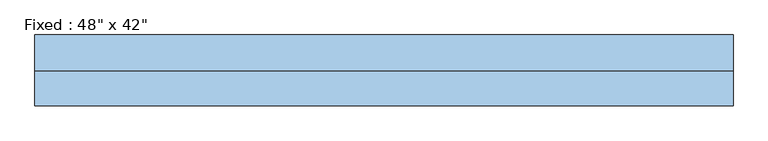
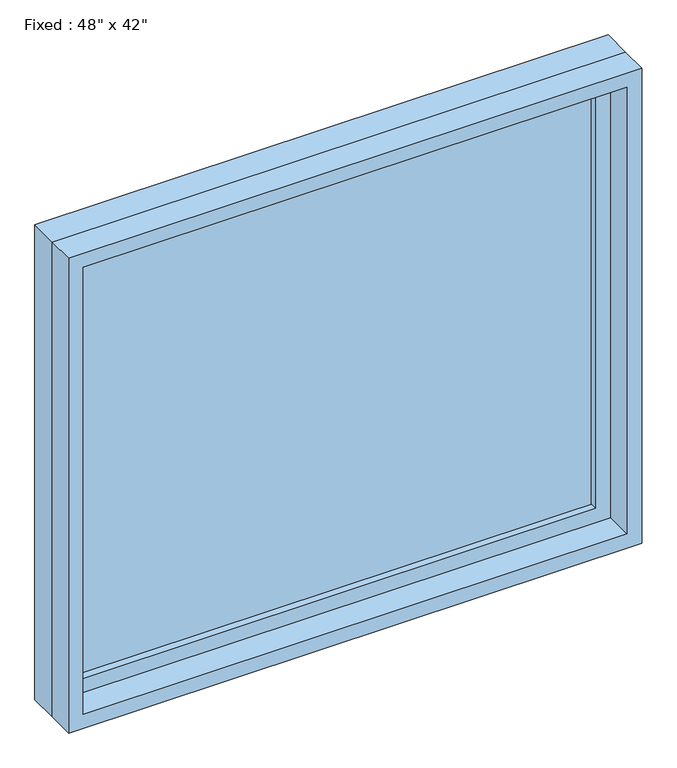
"""IFC4 building model written with IfcOpenShell, lengths in millimetres: window geometry."""

import ifcopenshell
import ifcopenshell.guid

model = None  # the IFC model being written
_history = None  # IfcOwnerHistory: only IFC2X3 demands one
_inside = {}  # id of a spatial element -> (the spatial element, [elements in it])
_under = {}  # id of a project, library or spatial element -> (it, [spatial elements below it])
_declared = {}  # id of a project -> (the project, [libraries it declares])
_typed = {}  # id of a type object -> (the type object, [elements of that type])
_made_of = {}  # id of a material, layer set ... -> (it, [elements and type objects made of it])


def new_model(schema):
    """Start an empty IFC model of exactly this schema.

    Asked for "IFC4X3", IfcOpenShell would pick the latest addendum, in which some entities
    have other attributes; the version numbers below select the first issue.
    IFC2X3 requires an IfcOwnerHistory on every rooted entity: one is made here for all.
    """
    global model, _history
    if schema == "IFC4X3":
        model = ifcopenshell.file(schema_version=(4, 3, 0, 0))
    else:
        model = ifcopenshell.file(schema=schema)
    _inside.clear()
    _under.clear()
    _declared.clear()
    _typed.clear()
    _made_of.clear()
    _history = None
    if model.schema == "IFC2X3":
        org = make("IfcOrganization", Name="unknown")
        user = make(
            "IfcPersonAndOrganization",
            ThePerson=make("IfcPerson", FamilyName="unknown"),
            TheOrganization=org,
        )
        app = make(
            "IfcApplication",
            ApplicationDeveloper=org,
            Version="unknown",
            ApplicationFullName="unknown",
            ApplicationIdentifier="unknown",
        )
        _history = make(
            "IfcOwnerHistory",
            OwningUser=user,
            OwningApplication=app,
            ChangeAction="ADDED",
            CreationDate=0,
        )
    return model


def make(cls, **values):
    """One entity of the class cls with the attributes given. An attribute that is None is left unset."""
    return model.create_entity(
        cls, **{name: value for name, value in values.items() if value is not None}
    )


def rooted(cls, **values):
    """An entity with a GlobalId (a new one), such as an element, a storey or a relation."""
    return make(cls, GlobalId=ifcopenshell.guid.new(), OwnerHistory=_history, **values)


def si_unit(unit_type, name, prefix=None):
    """IfcSIUnit, for example si_unit("LENGTHUNIT", "METRE", prefix="MILLI")."""
    return make("IfcSIUnit", UnitType=unit_type, Prefix=prefix, Name=name)


def assignment(units):
    """IfcUnitAssignment: the units of a project."""
    return None if units is None else make("IfcUnitAssignment", Units=units)


def point(xyz):
    """IfcCartesianPoint."""
    return None if xyz is None else make("IfcCartesianPoint", Coordinates=xyz)


def direction(xyz):
    """IfcDirection."""
    return None if xyz is None else make("IfcDirection", DirectionRatios=xyz)


def frame(location, z_axis=None, x_axis=None):
    """IfcAxis2Placement3D, a coordinate frame: its origin and axes. An axis left out is left unset."""
    return make(
        "IfcAxis2Placement3D",
        Location=point(location),
        Axis=direction(z_axis),
        RefDirection=direction(x_axis),
    )


def origin():
    """The frame at (0, 0, 0) with its axes left unset."""
    return frame((0.0, 0.0, 0.0))


def place(relative_to, where):
    """IfcLocalPlacement: puts the frame where relative to a parent placement (None: the world)."""
    return make(
        "IfcLocalPlacement", PlacementRelTo=relative_to, RelativePlacement=where
    )


def context(
    kind, dimensions, precision=None, world=None, true_north=None, identifier=None
):
    """IfcGeometricRepresentationContext, for example the 3D "Model" context."""
    return make(
        "IfcGeometricRepresentationContext",
        ContextIdentifier=identifier,
        ContextType=kind,
        CoordinateSpaceDimension=dimensions,
        Precision=precision,
        WorldCoordinateSystem=world,
        TrueNorth=true_north,
    )


def project(units=None, contexts=None):
    """IfcProject with its units and contexts."""
    return rooted(
        "IfcProject",
        Name="project",
        RepresentationContexts=contexts,
        UnitsInContext=assignment(units),
    )


def spatial(cls, under=None, at=None, **own):
    """A site, building, storey or space (cls), placed at a placement, below another one or the project."""
    s = rooted(cls, ObjectPlacement=at, **own)
    if under is not None:
        _under.setdefault(under.id(), (under, []))[1].append(s)
    return s


def polyline(points):
    """IfcPolyline through the points."""
    return make("IfcPolyline", Points=[point(p) for p in points])


def outline(outer, holes=None, kind="AREA"):
    """IfcArbitraryClosedProfileDef: a profile drawn as a closed curve; with holes, ...WithVoids."""
    if holes is None:
        return make("IfcArbitraryClosedProfileDef", ProfileType=kind, OuterCurve=outer)
    return make(
        "IfcArbitraryProfileDefWithVoids",
        ProfileType=kind,
        OuterCurve=outer,
        InnerCurves=holes,
    )


def extrude(swept, where, along, depth):
    """IfcExtrudedAreaSolid: the profile swept, set in the frame where, extruded along a direction by depth."""
    return make(
        "IfcExtrudedAreaSolid",
        SweptArea=swept,
        Position=where,
        ExtrudedDirection=direction(along),
        Depth=depth,
    )


def shape(context_of_items, identifier, shape_type, items):
    """IfcShapeRepresentation: the items that make up one representation, for example the "Body"."""
    return make(
        "IfcShapeRepresentation",
        ContextOfItems=context_of_items,
        RepresentationIdentifier=identifier,
        RepresentationType=shape_type,
        Items=items,
    )


def source(mapping_origin, context_of_items, identifier, shape_type, items):
    """IfcRepresentationMap: a shape defined once, which mapped items show again and again."""
    return make(
        "IfcRepresentationMap",
        MappingOrigin=mapping_origin,
        MappedRepresentation=shape(context_of_items, identifier, shape_type, items),
    )


def transform(
    local_origin,
    x_axis=None,
    y_axis=None,
    z_axis=None,
    scale=None,
    scale2=None,
    scale3=None,
    uniform=True,
):
    """IfcCartesianTransformationOperator3D, or its non-uniform kind. x_axis, y_axis, z_axis: its Axis1, 2, 3."""
    if uniform:
        return make(
            "IfcCartesianTransformationOperator3D",
            Axis1=direction(x_axis),
            Axis2=direction(y_axis),
            LocalOrigin=point(local_origin),
            Scale=scale,
            Axis3=direction(z_axis),
        )
    return make(
        "IfcCartesianTransformationOperator3DnonUniform",
        Axis1=direction(x_axis),
        Axis2=direction(y_axis),
        LocalOrigin=point(local_origin),
        Scale=scale,
        Axis3=direction(z_axis),
        Scale2=scale2,
        Scale3=scale3,
    )


def mapped(mapping_source, mapping_target):
    """IfcMappedItem: shows the shape of a source again, moved by a transform."""
    return make(
        "IfcMappedItem", MappingSource=mapping_source, MappingTarget=mapping_target
    )


def made_of(thing, what):
    """Note that an element or type object is made of a material, layer set ...; save() writes the relation."""
    if what is not None:
        _made_of.setdefault(what.id(), (what, []))[1].append(thing)
    return thing


def element(
    cls,
    number,
    at=None,
    inside=None,
    cuts=None,
    type_object=None,
    material=None,
    context=None,
    identifier="Body",
    shape_type=None,
    held_by="IfcProductDefinitionShape",
    body=None,
    shapes=None,
    **own,
):
    """One element of the class cls, such as IfcWall. Its Tag is "e" and its number.

    at: its placement. inside: the storey or other place that contains it. cuts: it is an
    opening in that element (IfcRelVoidsElement). A single representation is given by context,
    identifier, shape_type and body (its items); several are given by shapes. held_by: the class
    of the entity that holds the representations. save() writes the other relations.
    """
    e = rooted(cls, Tag="e%d" % number, ObjectPlacement=at, **own)
    if body is not None:
        shapes = [shape(context, identifier, shape_type, body)]
    if shapes is not None:
        e.Representation = make(held_by, Representations=shapes)
    if inside is not None:
        _inside.setdefault(inside.id(), (inside, []))[1].append(e)
    if cuts is not None:
        rooted(
            "IfcRelVoidsElement", RelatingBuildingElement=cuts, RelatedOpeningElement=e
        )
    if type_object is not None:
        _typed.setdefault(type_object.id(), (type_object, []))[1].append(e)
    return made_of(e, material)


def aggregate(whole, parts):
    """IfcRelAggregates: a whole, such as a stair, and the parts it consists of."""
    return rooted("IfcRelAggregates", RelatingObject=whole, RelatedObjects=parts)


def save(model, path):
    """Write the relations noted so far, then the file.

    IfcRelAggregates (storeys below a building ...), IfcRelContainedInSpatialStructure (elements
    in a storey), IfcRelDefinesByType, IfcRelAssociatesMaterial and IfcRelDeclares: one each for
    every whole, place, type object, material and project.
    """
    for whole, parts in _under.values():
        aggregate(whole, parts)
    for where, things in _inside.values():
        rooted(
            "IfcRelContainedInSpatialStructure",
            RelatedElements=things,
            RelatingStructure=where,
        )
    for kind, things in _typed.values():
        rooted("IfcRelDefinesByType", RelatedObjects=things, RelatingType=kind)
    for what, things in _made_of.values():
        rooted("IfcRelAssociatesMaterial", RelatedObjects=things, RelatingMaterial=what)
    for by, libraries in _declared.values():
        rooted("IfcRelDeclares", RelatingContext=by, RelatedDefinitions=libraries)
    model.write(path)


def window_b58e5159(model_context):
    return source(origin(), model_context, "Body", "SweptSolid", [
        extrude(outline(polyline([(508.0, 14.2875), (-584.2, 14.2875), (-584.2, 26.9875), (508.0, 26.9875), (508.0, 14.2875)])), frame((0.0, 0.0, 977.9), z_axis=(0.0, 0.0, 1.0), x_axis=(1.0, 0.0, 0.0)), (0.0, 0.0, 1.0), 939.8),
        extrude(outline(polyline([(1962.15, -628.65), (933.45, -628.65), (933.45, 552.45), (1962.15, 552.45), (1962.15, -628.65)]), holes=[polyline([(1917.7, -584.2), (1917.7, 508.0), (977.9, 508.0), (977.9, -584.2), (1917.7, -584.2)])]), frame((0.0, -1.5875, 0.0), z_axis=(0.0, 1.0, 0.0), x_axis=(0.0, 0.0, 1.0)), (0.0, 0.0, 1.0), 44.45),
        extrude(outline(polyline([(1981.2, -647.7), (914.4, -647.7), (914.4, 571.5), (1981.2, 571.5), (1981.2, -647.7)]), holes=[polyline([(1949.45, -615.95), (1949.45, 539.75), (946.15, 539.75), (946.15, -615.95), (1949.45, -615.95)])]), frame((0.0, -61.9125, 0.0), z_axis=(0.0, 1.0, 0.0), x_axis=(0.0, 0.0, 1.0)), (0.0, 0.0, 1.0), 60.325),
        extrude(outline(polyline([(1981.2, 571.5), (1981.2, -647.7), (914.4, -647.7), (914.4, 571.5), (1981.2, 571.5)]), holes=[polyline([(1962.15, 552.45), (933.45, 552.45), (933.45, -628.65), (1962.15, -628.65), (1962.15, 552.45)])]), frame((0.0, -1.5875, 0.0), z_axis=(0.0, 1.0, 0.0), x_axis=(0.0, 0.0, 1.0)), (0.0, 0.0, 1.0), 63.5),
    ])


if __name__ == "__main__":
    model = new_model("IFC4")
    model_context = context("Model", 3, world=origin())
    ifc_project = project(units=[si_unit("LENGTHUNIT", "METRE", prefix="MILLI")], contexts=[model_context])
    site = spatial("IfcSite", under=ifc_project)
    building = spatial("IfcBuilding", under=site)
    placement = place(None, origin())
    window_shape = window_b58e5159(model_context)
    element("IfcWindow", 1, ObjectType="Fixed : 48\" x 42\"", at=placement, inside=building, context=model_context, shape_type="MappedRepresentation", body=[
        mapped(window_shape, transform((0.0, 0.0, 0.0), x_axis=(1.0, 0.0, 0.0), y_axis=(0.0, 1.0, 0.0), z_axis=(0.0, 0.0, 1.0))),
    ])
    save(model, "model.ifc")

# Revit data of these elements
# Type "Fixed : 48\" x 42\""
#   Type Mark = "11"
#   Assembly Code = "B2020100"
#   Height = 3' - 6"
#   Default Sill Height = 3' - 0"
#   Width = 4' - 0"
#   Window Inset = 0' - 0 3/4"
#   Glass Pane Material = Glass
#   Sash Material = Sash
#   Wall Closure = (empty or 0)
# Element 1 (IfcWindow, "Fixed : 48\" x 42\"")
#   Materials on its faces: "Sash", "Glass"
# Materials
#   "Glass": class "Glass", colour RGB 0 128 192, transparency 0.75
#   "Sash": class "Wood", colour RGB 224 178 126, transparency 0
